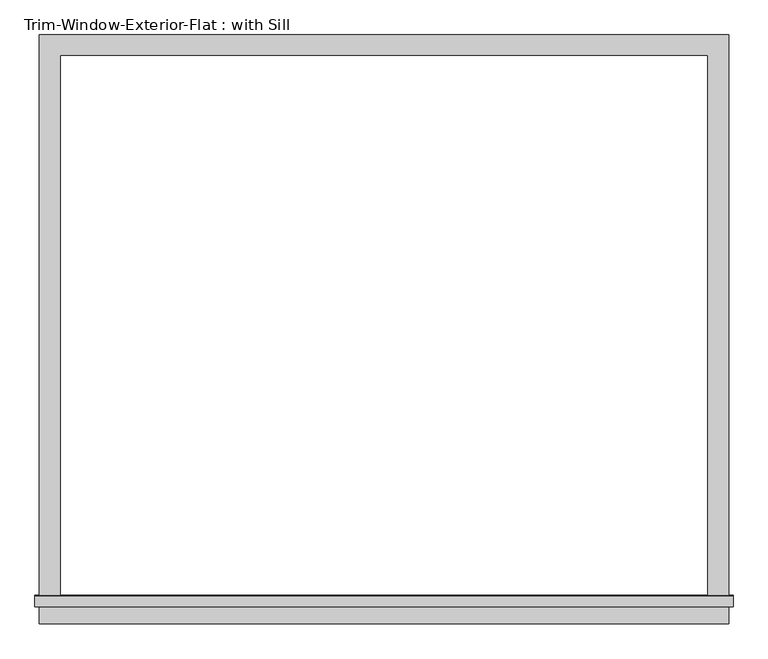
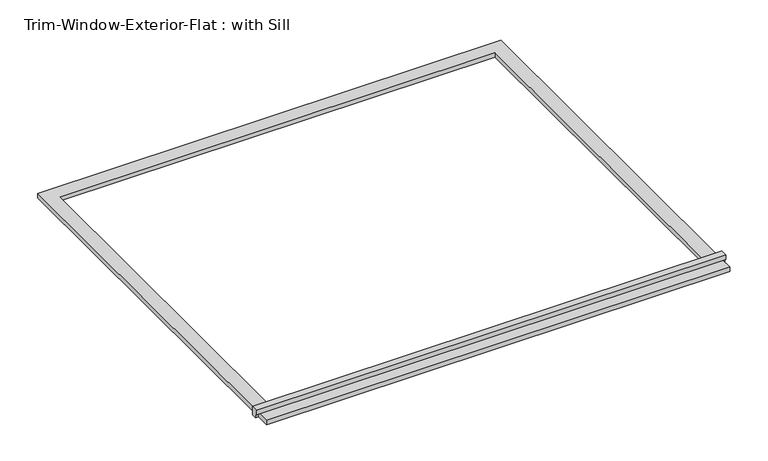
"""IFC4 building model written with IfcOpenShell, lengths in millimetres: proxy geometry, Trim-Window-Exterior-Flat : with Sill."""

from ifc_helpers import new_model, si_unit, frame, origin, origin_with_axes, place, context, project, spatial, polyline, outline, extrude, source, transform, mapped, element, save


def trim_window_exterior_flat_with_sill_86d3e75c(model_context):
    return source(origin(), model_context, "Body", "SweptSolid", [
        extrude(outline(polyline([(957.15, -1522.1823709), (957.15, -1579.3323709), (-957.15, -1579.3323709), (-957.15, -1522.1823709), (957.15, -1522.1823709)])), origin_with_axes(), (0.0, 0.0, 1.0), 19.05),
        extrude(outline(polyline([(-1531.75, 38.1), (-1502.4580645, 38.1), (-1500.0, 19.05), (-1500.0, 0.0), (-1522.1823709, 0.0), (-1522.1823709, 19.05), (-1531.75, 19.05), (-1531.75, 38.1)])), frame((-969.85, 0.0, 0.0), z_axis=(1.0, 0.0, 0.0), x_axis=(0.0, 1.0, 0.0)), (0.0, 0.0, 1.0), 1939.7),
        extrude(outline(polyline([(-957.15, 57.15), (957.15, 57.15), (957.15, -1500.0), (900.0, -1500.0), (900.0, 0.0), (-900.0, 0.0), (-900.0, -1500.0), (-957.15, -1500.0), (-957.15, 57.15)])), origin_with_axes(), (0.0, 0.0, 1.0), 19.05),
    ])


if __name__ == "__main__":
    model = new_model("IFC4")
    model_context = context("Model", 3, world=origin())
    ifc_project = project(units=[si_unit("LENGTHUNIT", "METRE", prefix="MILLI")], contexts=[model_context])
    site = spatial("IfcSite", under=ifc_project)
    building = spatial("IfcBuilding", under=site)
    placement = place(None, origin())
    trim_window_exterior_flat_with_sill_shape = trim_window_exterior_flat_with_sill_86d3e75c(model_context)
    element("IfcBuildingElementProxy", 1, Name="Trim-Window-Exterior-Flat : with Sill", ObjectType="Trim-Window-Exterior-Flat : with Sill", at=placement, inside=building, context=model_context, shape_type="MappedRepresentation", body=[
        mapped(trim_window_exterior_flat_with_sill_shape, transform((0.0, 0.0, 0.0), x_axis=(1.0, 0.0, 0.0), y_axis=(0.0, 1.0, 0.0), z_axis=(0.0, 0.0, 1.0))),
    ])
    save(model, "model.ifc")

# Revit data of these elements
# Type "Trim-Window-Exterior-Flat : with Sill"
#   Trim Width = 5.715 cm
#   Trim Thickness_Picture Frame = 3.175 cm
#   Trim Thickness_with Sill = 1.905 cm
#   Sill Thickness = 3.175 cm
#   Opening Width [instance default] = 60.96 cm
#   Opening Height [instance default] = 91.44 cm
#   Default Elevation = 121.92 cm
#   Sill = yes
#   Picture Frame = no
#   Trim Material [instance default] = none
# Element 1 (IfcBuildingElementProxy, "Trim-Window-Exterior-Flat : with Sill")
#   Opening Width = 180 cm
#   Opening Height = 150 cm
#   Trim Material = Clad - White
#   Materials on its faces: "Clad - White"
# Materials
#   "Clad - White": class "Wood", colour RGB 242 242 238, transparency 0, Cost = 0
